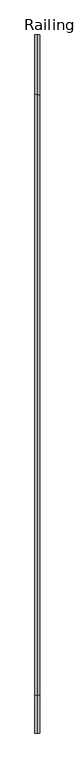
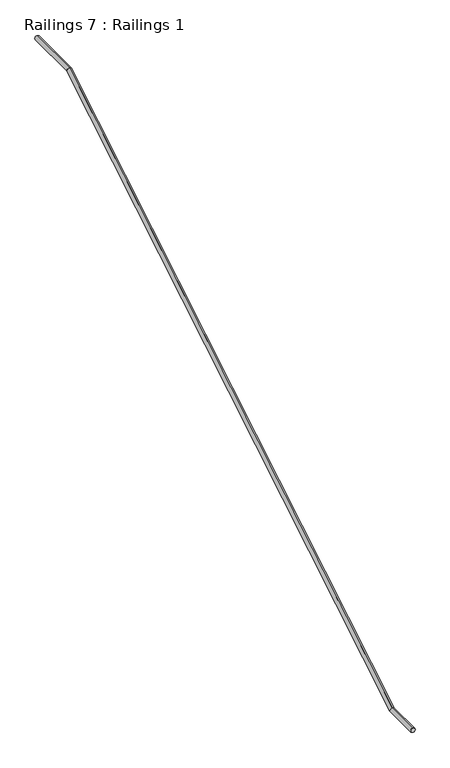
"""IFC4 building model written with IfcOpenShell, lengths in millimetres: railing geometry, Railings 7 : Railings 1."""

from ifc_helpers import new_model, si_unit, frame, origin, place, context, project, spatial, circle_curve, ellipse_curve, source, transform, mapped, element, save
from ifc_brep_helpers import plane_surface, cylinder_surface, advanced_brep


def railings_7_railings_1_b0177f6f(model_context):
    return source(origin(), model_context, "Body", "AdvancedBrep", [
        advanced_brep(
        [(32273.1661999, 35367.7792286, 270087.725), (32273.1661999, 35367.7792286, 270125.825), (32273.1661999, 29843.4168167, 267230.225), (32273.1661999, 29843.4168167, 267268.325), (32273.1661999, 34903.3054525, 270087.725), (32273.1661999, 34892.7281809, 270125.825), (32273.1661999, 30153.5054525, 267230.225), (32273.1661999, 30142.9281809, 267268.325)],
        [
            (0, 1, circle_curve(frame((32273.1661999, 35367.7792286, 270106.775), z_axis=(0.0, 1.0, 0.0), x_axis=(0.0, 0.0, 1.0)), 19.05)),
            (1, 0, circle_curve(frame((32273.1661999, 35367.7792286, 270106.775), z_axis=(0.0, 1.0, 0.0), x_axis=(0.0, 0.0, 1.0)), 19.05)),
            (2, 3, circle_curve(frame((32273.1661999, 29843.4168167, 267249.275), z_axis=(0.0, -1.0, 0.0), x_axis=(0.0, 0.0, 1.0)), 19.05)),
            (3, 2, circle_curve(frame((32273.1661999, 29843.4168167, 267249.275), z_axis=(0.0, -1.0, 0.0), x_axis=(0.0, 0.0, 1.0)), 19.05)),
            (0, 4),
            (4, 5, ellipse_curve(frame((32273.1661999, 34898.0168167, 270106.775), z_axis=(0.0, 0.9635574326636285, 0.2675015401052433), x_axis=(0.0, 0.26750154010524313, -0.9635574326636285)), 19.7704873, 19.05)),
            (5, 1),
            (5, 4, ellipse_curve(frame((32273.1661999, 34898.0168167, 270106.775), z_axis=(0.0, 0.9635574326636285, 0.2675015401052433), x_axis=(0.0, 0.26750154010524313, -0.9635574326636285)), 19.7704873, 19.05)),
            (4, 6),
            (6, 7, ellipse_curve(frame((32273.1661999, 30148.2168167, 267249.275), z_axis=(0.0, 0.9635574326636285, 0.2675015401052433), x_axis=(0.0, -0.2675015401052434, 0.9635574326636284)), 19.7704873, 19.05)),
            (7, 5),
            (7, 6, ellipse_curve(frame((32273.1661999, 30148.2168167, 267249.275), z_axis=(0.0, 0.9635574326636285, 0.2675015401052433), x_axis=(0.0, -0.2675015401052434, 0.9635574326636284)), 19.7704873, 19.05)),
            (6, 2),
            (3, 7),
        ],
        [
            plane_surface(frame((32292.2161999, 35367.7792286, 270106.775), z_axis=(0.0, 1.0, 0.0), x_axis=(1.0, 0.0, 0.0))),
            plane_surface(frame((32292.2161999, 29843.4168167, 267249.275), z_axis=(0.0, -1.0, 0.0), x_axis=(1.0, 0.0, 0.0))),
            cylinder_surface(frame((32273.1661999, 35367.7792286, 270106.775), z_axis=(0.0, 1.0, 0.0), x_axis=(0.0, 0.0, 1.0)), 19.05),
            cylinder_surface(frame((32273.1661999, 34898.0168167, 270106.775), z_axis=(0.0, 0.8568858520826458, 0.5155061944347499), x_axis=(0.0, -0.5155061944347499, 0.8568858520826458)), 19.05),
            cylinder_surface(frame((32273.1661999, 30148.2168167, 267249.275), z_axis=(0.0, 1.0, 0.0), x_axis=(0.0, 0.0, 1.0)), 19.05),
        ],
        [
            (0, [[1, 2]]),
            (1, [[3, 4]]),
            (2, [[-1, 5, 6, 7]]),
            (2, [[-2, -7, 8, -5]]),
            (3, [[-6, 9, 10, 11]]),
            (3, [[-8, -11, 12, -9]]),
            (4, [[-10, 13, -4, 14]]),
            (4, [[-12, -14, -3, -13]]),
        ],
    ),
    ])


if __name__ == "__main__":
    model = new_model("IFC4")
    model_context = context("Model", 3, world=origin())
    ifc_project = project(units=[si_unit("LENGTHUNIT", "METRE", prefix="MILLI")], contexts=[model_context])
    site = spatial("IfcSite", under=ifc_project)
    building = spatial("IfcBuilding", under=site)
    placement = place(None, origin())
    railings_7_railings_1_shape = railings_7_railings_1_b0177f6f(model_context)
    element("IfcRailing", 1, ObjectType="Railings 7 : Railings 1", at=placement, inside=building, context=model_context, shape_type="MappedRepresentation", body=[
        mapped(railings_7_railings_1_shape, transform((0.0, 0.0, 0.0), x_axis=(1.0, 0.0, 0.0), y_axis=(0.0, 1.0, 0.0), z_axis=(0.0, 0.0, 1.0))),
    ])
    save(model, "model.ifc")

# Revit data of these elements
# Element 1 (IfcRailing, "Railings 7 : Railings 1")
#   Materials on its faces: "ALUM. RAILING"
# Materials
#   "ALUM. RAILING": class "Generic", colour RGB 255 255 255, transparency 0, Cost = 0
